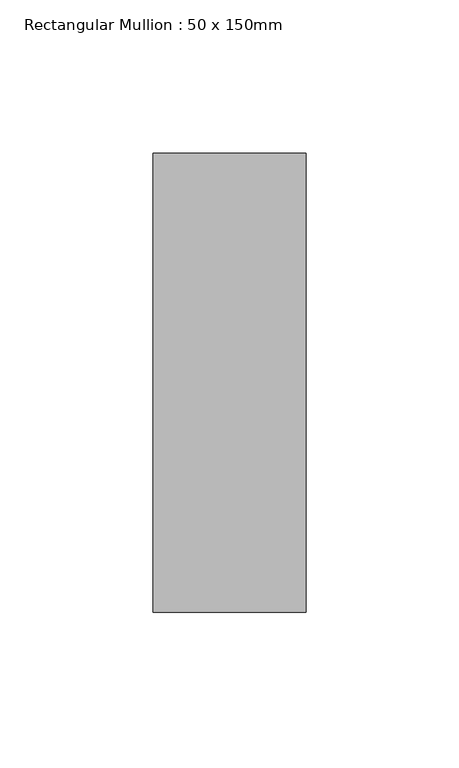
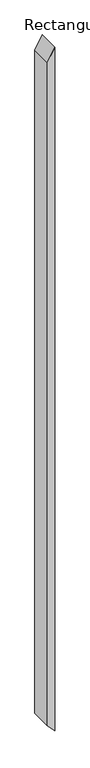
"""IFC4 building model written with IfcOpenShell, lengths in millimetres: member geometry, Rectangular Mullion : 50 x 150mm."""

from ifc_helpers import new_model, si_unit, frame, origin, place, context, project, spatial, polyline, outline, extrude, source, transform, mapped, element, save


def rectangular_mullion_50_x_150mm_5a0cd9cb(model_context):
    return source(origin(), model_context, "Body", "SweptSolid", [
        extrude(outline(polyline([(0.0, 0.0), (-92.7617394, -50.0), (-4930.0822697, -50.0), (-4983.1907154, 0.0), (0.0, 0.0)])), frame((0.0, -75.0, 0.0), z_axis=(0.0, 1.0, 0.0), x_axis=(0.0, 0.0, 1.0)), (0.0, 0.0, 1.0), 150.0),
    ])


if __name__ == "__main__":
    model = new_model("IFC4")
    model_context = context("Model", 3, world=origin())
    ifc_project = project(units=[si_unit("LENGTHUNIT", "METRE", prefix="MILLI")], contexts=[model_context])
    site = spatial("IfcSite", under=ifc_project)
    building = spatial("IfcBuilding", under=site)
    placement = place(None, origin())
    rectangular_mullion_50_x_150mm_shape = rectangular_mullion_50_x_150mm_5a0cd9cb(model_context)
    element("IfcMember", 1, ObjectType="Rectangular Mullion : 50 x 150mm", at=placement, inside=building, context=model_context, shape_type="MappedRepresentation", body=[
        mapped(rectangular_mullion_50_x_150mm_shape, transform((0.0, 0.0, 0.0), x_axis=(1.0, 0.0, 0.0), y_axis=(0.0, 1.0, 0.0), z_axis=(0.0, 0.0, 1.0))),
    ])
    save(model, "model.ifc")

# Revit data of these elements
# Type "Rectangular Mullion : 50 x 150mm"
#   built-in parameter 1007304 = 0.492126 (stored number, unit not read)
#   built-in parameter 1007301 = 0.082021 (stored number, unit not read)
#   built-in parameter 1007300 = 0.082021 (stored number, unit not read)
# Element 1 (IfcMember, "Rectangular Mullion : 50 x 150mm")
#   Materials on its faces: "Metal - Aluminium"
# Materials
#   "Metal - Aluminium": class "Metal", colour RGB 247 247 247, transparency 0
